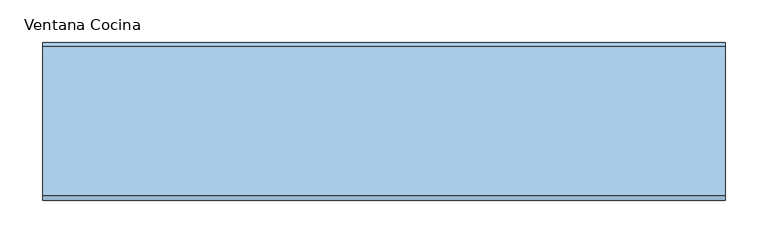
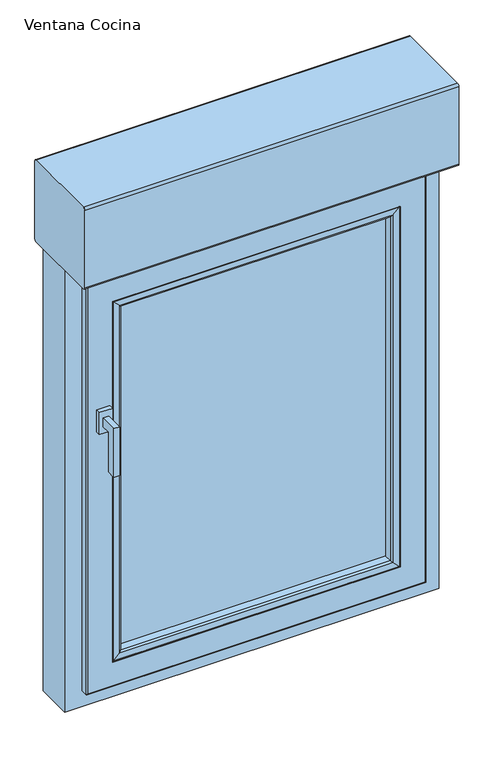
"""IFC4 building model written with IfcOpenShell, lengths in millimetres: window geometry, 2019_ES_Ventana_Replus_re80pvc301_10100_box_1-Hoja_con-Compacto : Ventana Cocina."""

import ifcopenshell
import ifcopenshell.guid

model = None  # the IFC model being written
_history = None  # IfcOwnerHistory: only IFC2X3 demands one
_inside = {}  # id of a spatial element -> (the spatial element, [elements in it])
_under = {}  # id of a project, library or spatial element -> (it, [spatial elements below it])
_declared = {}  # id of a project -> (the project, [libraries it declares])
_typed = {}  # id of a type object -> (the type object, [elements of that type])
_made_of = {}  # id of a material, layer set ... -> (it, [elements and type objects made of it])


def new_model(schema):
    """Start an empty IFC model of exactly this schema.

    Asked for "IFC4X3", IfcOpenShell would pick the latest addendum, in which some entities
    have other attributes; the version numbers below select the first issue.
    IFC2X3 requires an IfcOwnerHistory on every rooted entity: one is made here for all.
    """
    global model, _history
    if schema == "IFC4X3":
        model = ifcopenshell.file(schema_version=(4, 3, 0, 0))
    else:
        model = ifcopenshell.file(schema=schema)
    _inside.clear()
    _under.clear()
    _declared.clear()
    _typed.clear()
    _made_of.clear()
    _history = None
    if model.schema == "IFC2X3":
        org = make("IfcOrganization", Name="unknown")
        user = make(
            "IfcPersonAndOrganization",
            ThePerson=make("IfcPerson", FamilyName="unknown"),
            TheOrganization=org,
        )
        app = make(
            "IfcApplication",
            ApplicationDeveloper=org,
            Version="unknown",
            ApplicationFullName="unknown",
            ApplicationIdentifier="unknown",
        )
        _history = make(
            "IfcOwnerHistory",
            OwningUser=user,
            OwningApplication=app,
            ChangeAction="ADDED",
            CreationDate=0,
        )
    return model


def make(cls, **values):
    """One entity of the class cls with the attributes given. An attribute that is None is left unset."""
    return model.create_entity(
        cls, **{name: value for name, value in values.items() if value is not None}
    )


def rooted(cls, **values):
    """An entity with a GlobalId (a new one), such as an element, a storey or a relation."""
    return make(cls, GlobalId=ifcopenshell.guid.new(), OwnerHistory=_history, **values)


def si_unit(unit_type, name, prefix=None):
    """IfcSIUnit, for example si_unit("LENGTHUNIT", "METRE", prefix="MILLI")."""
    return make("IfcSIUnit", UnitType=unit_type, Prefix=prefix, Name=name)


def assignment(units):
    """IfcUnitAssignment: the units of a project."""
    return None if units is None else make("IfcUnitAssignment", Units=units)


def point(xyz):
    """IfcCartesianPoint."""
    return None if xyz is None else make("IfcCartesianPoint", Coordinates=xyz)


def direction(xyz):
    """IfcDirection."""
    return None if xyz is None else make("IfcDirection", DirectionRatios=xyz)


def frame(location, z_axis=None, x_axis=None):
    """IfcAxis2Placement3D, a coordinate frame: its origin and axes. An axis left out is left unset."""
    return make(
        "IfcAxis2Placement3D",
        Location=point(location),
        Axis=direction(z_axis),
        RefDirection=direction(x_axis),
    )


def frame_2d(location, x_axis=None):
    """IfcAxis2Placement2D, a coordinate frame in the plane: its origin and x axis."""
    return make(
        "IfcAxis2Placement2D", Location=point(location), RefDirection=direction(x_axis)
    )


def origin():
    """The frame at (0, 0, 0) with its axes left unset."""
    return frame((0.0, 0.0, 0.0))


def place(relative_to, where):
    """IfcLocalPlacement: puts the frame where relative to a parent placement (None: the world)."""
    return make(
        "IfcLocalPlacement", PlacementRelTo=relative_to, RelativePlacement=where
    )


def context(
    kind, dimensions, precision=None, world=None, true_north=None, identifier=None
):
    """IfcGeometricRepresentationContext, for example the 3D "Model" context."""
    return make(
        "IfcGeometricRepresentationContext",
        ContextIdentifier=identifier,
        ContextType=kind,
        CoordinateSpaceDimension=dimensions,
        Precision=precision,
        WorldCoordinateSystem=world,
        TrueNorth=true_north,
    )


def project(units=None, contexts=None):
    """IfcProject with its units and contexts."""
    return rooted(
        "IfcProject",
        Name="project",
        RepresentationContexts=contexts,
        UnitsInContext=assignment(units),
    )


def spatial(cls, under=None, at=None, **own):
    """A site, building, storey or space (cls), placed at a placement, below another one or the project."""
    s = rooted(cls, ObjectPlacement=at, **own)
    if under is not None:
        _under.setdefault(under.id(), (under, []))[1].append(s)
    return s


def polyline(points):
    """IfcPolyline through the points."""
    return make("IfcPolyline", Points=[point(p) for p in points])


def circle_curve(where, radius):
    """IfcCircle in the frame where."""
    return make("IfcCircle", Position=where, Radius=radius)


def ellipse_curve(where, semi_axis1, semi_axis2):
    """IfcEllipse in the frame where."""
    return make(
        "IfcEllipse", Position=where, SemiAxis1=semi_axis1, SemiAxis2=semi_axis2
    )


def trimmed(basis, trim1, trim2, sense, master):
    """IfcTrimmedCurve: the piece of a basis curve between two trims."""
    return make(
        "IfcTrimmedCurve",
        BasisCurve=basis,
        Trim1=trim1,
        Trim2=trim2,
        SenseAgreement=sense,
        MasterRepresentation=master,
    )


def segment(curve, same_sense, transition):
    """IfcCompositeCurveSegment."""
    return make(
        "IfcCompositeCurveSegment",
        Transition=transition,
        SameSense=same_sense,
        ParentCurve=curve,
    )


def composite_curve(segments, self_intersect=None):
    """IfcCompositeCurve: segments joined end to end."""
    return make("IfcCompositeCurve", Segments=segments, SelfIntersect=self_intersect)


def outline(outer, holes=None, kind="AREA"):
    """IfcArbitraryClosedProfileDef: a profile drawn as a closed curve; with holes, ...WithVoids."""
    if holes is None:
        return make("IfcArbitraryClosedProfileDef", ProfileType=kind, OuterCurve=outer)
    return make(
        "IfcArbitraryProfileDefWithVoids",
        ProfileType=kind,
        OuterCurve=outer,
        InnerCurves=holes,
    )


def extrude(swept, where, along, depth):
    """IfcExtrudedAreaSolid: the profile swept, set in the frame where, extruded along a direction by depth."""
    return make(
        "IfcExtrudedAreaSolid",
        SweptArea=swept,
        Position=where,
        ExtrudedDirection=direction(along),
        Depth=depth,
    )


def shape(context_of_items, identifier, shape_type, items):
    """IfcShapeRepresentation: the items that make up one representation, for example the "Body"."""
    return make(
        "IfcShapeRepresentation",
        ContextOfItems=context_of_items,
        RepresentationIdentifier=identifier,
        RepresentationType=shape_type,
        Items=items,
    )


def source(mapping_origin, context_of_items, identifier, shape_type, items):
    """IfcRepresentationMap: a shape defined once, which mapped items show again and again."""
    return make(
        "IfcRepresentationMap",
        MappingOrigin=mapping_origin,
        MappedRepresentation=shape(context_of_items, identifier, shape_type, items),
    )


def transform(
    local_origin,
    x_axis=None,
    y_axis=None,
    z_axis=None,
    scale=None,
    scale2=None,
    scale3=None,
    uniform=True,
):
    """IfcCartesianTransformationOperator3D, or its non-uniform kind. x_axis, y_axis, z_axis: its Axis1, 2, 3."""
    if uniform:
        return make(
            "IfcCartesianTransformationOperator3D",
            Axis1=direction(x_axis),
            Axis2=direction(y_axis),
            LocalOrigin=point(local_origin),
            Scale=scale,
            Axis3=direction(z_axis),
        )
    return make(
        "IfcCartesianTransformationOperator3DnonUniform",
        Axis1=direction(x_axis),
        Axis2=direction(y_axis),
        LocalOrigin=point(local_origin),
        Scale=scale,
        Axis3=direction(z_axis),
        Scale2=scale2,
        Scale3=scale3,
    )


def mapped(mapping_source, mapping_target):
    """IfcMappedItem: shows the shape of a source again, moved by a transform."""
    return make(
        "IfcMappedItem", MappingSource=mapping_source, MappingTarget=mapping_target
    )


def made_of(thing, what):
    """Note that an element or type object is made of a material, layer set ...; save() writes the relation."""
    if what is not None:
        _made_of.setdefault(what.id(), (what, []))[1].append(thing)
    return thing


def element(
    cls,
    number,
    at=None,
    inside=None,
    cuts=None,
    type_object=None,
    material=None,
    context=None,
    identifier="Body",
    shape_type=None,
    held_by="IfcProductDefinitionShape",
    body=None,
    shapes=None,
    **own,
):
    """One element of the class cls, such as IfcWall. Its Tag is "e" and its number.

    at: its placement. inside: the storey or other place that contains it. cuts: it is an
    opening in that element (IfcRelVoidsElement). A single representation is given by context,
    identifier, shape_type and body (its items); several are given by shapes. held_by: the class
    of the entity that holds the representations. save() writes the other relations.
    """
    e = rooted(cls, Tag="e%d" % number, ObjectPlacement=at, **own)
    if body is not None:
        shapes = [shape(context, identifier, shape_type, body)]
    if shapes is not None:
        e.Representation = make(held_by, Representations=shapes)
    if inside is not None:
        _inside.setdefault(inside.id(), (inside, []))[1].append(e)
    if cuts is not None:
        rooted(
            "IfcRelVoidsElement", RelatingBuildingElement=cuts, RelatedOpeningElement=e
        )
    if type_object is not None:
        _typed.setdefault(type_object.id(), (type_object, []))[1].append(e)
    return made_of(e, material)


def aggregate(whole, parts):
    """IfcRelAggregates: a whole, such as a stair, and the parts it consists of."""
    return rooted("IfcRelAggregates", RelatingObject=whole, RelatedObjects=parts)


def save(model, path):
    """Write the relations noted so far, then the file.

    IfcRelAggregates (storeys below a building ...), IfcRelContainedInSpatialStructure (elements
    in a storey), IfcRelDefinesByType, IfcRelAssociatesMaterial and IfcRelDeclares: one each for
    every whole, place, type object, material and project.
    """
    for whole, parts in _under.values():
        aggregate(whole, parts)
    for where, things in _inside.values():
        rooted(
            "IfcRelContainedInSpatialStructure",
            RelatedElements=things,
            RelatingStructure=where,
        )
    for kind, things in _typed.values():
        rooted("IfcRelDefinesByType", RelatedObjects=things, RelatingType=kind)
    for what, things in _made_of.values():
        rooted("IfcRelAssociatesMaterial", RelatedObjects=things, RelatingMaterial=what)
    for by, libraries in _declared.values():
        rooted("IfcRelDeclares", RelatingContext=by, RelatedDefinitions=libraries)
    model.write(path)


def plane_surface(at):
    """IfcPlane: the flat surface through the origin of the frame at, square to its z axis."""
    return make("IfcPlane", Position=at)


def cylinder_surface(at, radius):
    """IfcCylindricalSurface: all points at the distance radius from the z axis of the frame at."""
    return make("IfcCylindricalSurface", Position=at, Radius=radius)


def advanced_brep(points, edges, surfaces, faces):
    """IfcAdvancedBrep: a solid bounded by faces that lie on surfaces and meet in shared edges.

    An edge is (start, end): straight between two places in points (the first is 0);
    or (start, end, curve); or (start, end, curve, False) where it runs against its curve.
    A face is (place in surfaces, loops), or (place, loops, False) where it looks against
    its surface's normal. A loop lists edges by number (the first is 1), with a minus sign
    where the edge is run from its end to its start. The first loop is the outer one.
    """
    corners = [point(p) for p in points]
    vertices = [make("IfcVertexPoint", VertexGeometry=c) for c in corners]
    made = []
    for start, end, *more in edges:
        made.append(
            make(
                "IfcEdgeCurve",
                EdgeStart=vertices[start],
                EdgeEnd=vertices[end],
                EdgeGeometry=more[0] if more else make("IfcPolyline", Points=[corners[start], corners[end]]),
                SameSense=more[1] if len(more) > 1 else True,
            )
        )
    hull = []
    for where, loops, *sense in faces:
        bounds = []
        for j, loop in enumerate(loops):
            ring = [make("IfcOrientedEdge", EdgeElement=made[abs(k) - 1], Orientation=k > 0) for k in loop]
            bounds.append(
                make(
                    "IfcFaceOuterBound" if j == 0 else "IfcFaceBound",
                    Bound=make("IfcEdgeLoop", EdgeList=ring),
                    Orientation=True,
                )
            )
        hull.append(make("IfcAdvancedFace", Bounds=bounds, FaceSurface=surfaces[where], SameSense=sense[0] if sense else True))
    return make("IfcAdvancedBrep", Outer=make("IfcClosedShell", CfsFaces=hull))


def ventana_cocina_c5497abf(model_context):
    return source(origin(), model_context, "Body", "SolidModel", [
        extrude(outline(composite_curve([segment(polyline([(55.0, 1810.0), (-120.0, 1810.0)]), True, "CONTINUOUS"), segment(trimmed(circle_curve(frame_2d((-120.0, 1815.0)), 5.0), [point((-120.0, 1810.0))], [point((-125.0, 1815.0))], False, "CARTESIAN"), True, "CONTINUOUS"), segment(polyline([(-125.0, 1815.0), (-125.0, 1990.0)]), True, "CONTINUOUS"), segment(trimmed(circle_curve(frame_2d((-120.0, 1990.0)), 5.0), [point((-125.0, 1990.0))], [point((-120.0, 1995.0))], False, "CARTESIAN"), True, "CONTINUOUS"), segment(polyline([(-120.0, 1995.0), (55.0, 1995.0)]), True, "CONTINUOUS"), segment(trimmed(circle_curve(frame_2d((55.0, 1990.0)), 5.0), [point((55.0, 1995.0))], [point((60.0, 1990.0))], False, "CARTESIAN"), True, "CONTINUOUS"), segment(polyline([(60.0, 1990.0), (60.0, 1815.0)]), True, "CONTINUOUS"), segment(trimmed(circle_curve(frame_2d((55.0, 1815.0)), 5.0), [point((60.0, 1815.0))], [point((55.0, 1810.0))], False, "CARTESIAN"), True, "CONTINUOUS")], self_intersect=False)), frame((-400.0, 0.0, 0.0), z_axis=(1.0, 0.0, 0.0), x_axis=(0.0, 1.0, 0.0)), (0.0, 0.0, 1.0), 800.0),
        extrude(outline(polyline([(-78.4999991, 1470.0), (-78.4999991, 1450.0), (-98.4999991, 1450.0), (-98.4999991, 1360.0), (-118.4999991, 1360.0), (-118.4999991, 1470.0), (-78.4999991, 1470.0)])), frame((-334.1999993, 0.0, 0.0), z_axis=(1.0, 0.0, 0.0), x_axis=(0.0, 1.0, 0.0)), (0.0, 0.0, 1.0), 12.0),
        extrude(outline(polyline([(-313.9687607, -78.4999991), (-342.4312378, -78.4999991), (-342.4312378, -68.4999991), (-313.9687607, -68.4999991), (-313.9687607, -78.4999991)])), frame((0.0, 0.0, 1435.217127), z_axis=(0.0, 0.0, 1.0), x_axis=(1.0, 0.0, 0.0)), (0.0, 0.0, 1.0), 49.565746),
        extrude(outline(polyline([(1707.2, 297.1999993), (1707.2, -297.1999993), (909.8, -297.1999993), (909.8, 297.1999993), (1707.2, 297.1999993)]), holes=[polyline([(917.8, 289.1999993), (917.8, -289.1999993), (1699.2, -289.1999993), (1699.2, 289.1999993), (917.8, 289.1999993)])]), frame((0.0, -26.9999999, 0.0), z_axis=(0.0, 1.0, 0.0), x_axis=(0.0, 0.0, 1.0)), (0.0, 0.0, 1.0), 16.0),
        extrude(outline(polyline([(1707.1868066, 297.1868058), (1707.1868066, -297.1868058), (909.8131934, -297.1868058), (909.8131934, 297.1868058), (1707.1868066, 297.1868058)]), holes=[polyline([(917.8, 289.1999993), (917.8, -289.1999993), (1699.2, -289.1999993), (1699.2, 289.1999993), (917.8, 289.1999993)])]), frame((0.0, -47.0000001, 0.0), z_axis=(0.0, 1.0, 0.0), x_axis=(0.0, 0.0, 1.0)), (0.0, 0.0, 1.0), 16.0),
        extrude(outline(polyline([(297.1999993, -6.9999997), (297.1999993, -10.9999999), (-297.1999993, -10.9999999), (-297.1999993, -6.9999997), (297.1999993, -6.9999997)])), frame((0.0, 0.0, 903.7946451), z_axis=(0.0, 0.0, 1.0), x_axis=(1.0, 0.0, 0.0)), (0.0, 0.0, 1.0), 809.4053549),
        extrude(outline(polyline([(297.1999993, -26.9999999), (297.1999993, -31.0000001), (-297.1999993, -31.0000001), (-297.1999993, -26.9999999), (297.1999993, -26.9999999)])), frame((0.0, 0.0, 903.7946451), z_axis=(0.0, 0.0, 1.0), x_axis=(1.0, 0.0, 0.0)), (0.0, 0.0, 1.0), 809.4053549),
        extrude(outline(polyline([(297.1999993, -47.0000001), (297.1999993, -51.0000003), (-297.1999993, -51.0000003), (-297.1999993, -47.0000001), (297.1999993, -47.0000001)])), frame((0.0, 0.0, 903.7946451), z_axis=(0.0, 0.0, 1.0), x_axis=(1.0, 0.0, 0.0)), (0.0, 0.0, 1.0), 809.4053549),
        advanced_brep(
        [(287.2913171, 9.2764571, 1697.2913178), (290.1890946, 11.5, 1700.1890953), (290.1890946, 11.5, 919.8109047), (287.2913171, 9.2764571, 922.7086822), (330.1999993, 11.5, 879.8), (-330.1999993, 11.5, 879.8), (-330.1999993, 11.5, 1740.2), (330.1999993, 11.5, 1740.2), (-290.1890946, 11.5, 1700.1890953), (-290.1890946, 11.5, 919.8109047), (-287.2913171, 9.2764571, 922.7086822), (284.1757968, -2.3508228, 1694.1757976), (284.1757968, -2.3508228, 925.8242024), (-284.1757968, -2.3508228, 925.8242024), (284.6739305, -3.0000033, 1694.6739313), (284.6739305, -3.0000033, 925.3260687), (-284.6739305, -3.0000033, 925.3260687), (291.1999993, -3.0000033, 1701.2), (-291.1999993, -3.0000033, 1701.2), (-291.1999993, -3.0000033, 918.8), (291.1999993, -3.0000033, 918.8), (-284.6739305, -3.0000033, 1694.6739313), (291.1999993, -6.9999997, 1701.2), (291.1999993, -6.9999997, 918.8), (-291.1999993, -6.9999997, 918.8), (311.8162192, -6.9999997, 1721.8162199), (-311.8162192, -6.9999997, 1721.8162199), (-311.8162192, -6.9999997, 898.1837801), (311.8162192, -6.9999997, 898.1837801), (-291.1999993, -6.9999997, 1701.2), (309.1999993, -25.6153717, 1719.2), (309.1999993, -25.6153717, 900.8), (-309.1999993, -25.6153717, 900.8), (309.1999993, -56.4999995, 1719.2), (309.1999993, -56.4999995, 900.8), (-309.1999993, -56.4999995, 900.8), (-309.1999993, -56.4999995, 1719.2), (297.1999993, -56.4999995, 1707.2), (-297.1999993, -56.4999995, 1707.2), (-297.1999993, -56.4999995, 912.8), (297.1999993, -56.4999995, 912.8), (297.1999993, -51.0000003, 1707.2), (297.1999993, -51.0000003, 912.8), (-297.1999993, -51.0000003, 912.8), (-297.1999993, -51.0000003, 1707.2), (286.007687, -51.0000003, 1696.0076877), (-286.007687, -51.0000003, 1696.0076877), (-286.007687, -51.0000003, 923.9923123), (286.007687, -51.0000003, 923.9923123), (285.4940999, -51.6693201, 1695.4941006), (285.4940999, -51.6693201, 924.5058994), (-285.4940999, -51.6693201, 924.5058994), (288.8993918, -64.3780426, 1698.8993925), (288.8993918, -64.3780426, 921.1006075), (-288.8993918, -64.3780426, 921.1006075), (292.6234971, -67.3403297, 1702.6234978), (292.6234971, -67.3403297, 917.3765022), (-292.6234971, -67.3403297, 917.3765022), (305.6488427, -67.7951848, 1715.6488434), (305.6488427, -67.7951848, 904.3511566), (-305.6488427, -67.7951848, 904.3511566), (306.1999993, -67.2629391, 1716.2), (306.1999993, -67.2629391, 903.8), (-306.1999993, -67.2629391, 903.8), (307.4370593, -68.4999991, 1717.43706), (307.4370593, -68.4999991, 902.56294), (-307.4370593, -68.4999991, 902.56294), (360.1999993, -68.4999991, 1770.2), (-360.1999993, -68.4999991, 1770.2), (-360.1999993, -68.4999991, 849.8), (360.1999993, -68.4999991, 849.8), (-307.4370593, -68.4999991, 1717.43706), (363.1999993, -65.4999991, 1773.2), (363.1999993, -65.4999991, 846.8), (-363.1999993, -65.4999991, 846.8), (363.1999993, -50.0, 1773.2), (363.1999993, -50.0, 846.8), (-363.1999993, -50.0, 846.8), (-363.1999993, -50.0, 1773.2), (343.1999993, -50.0, 1753.2), (-343.1999993, -50.0, 1753.2), (-343.1999993, -50.0, 866.8), (343.1999993, -50.0, 866.8), (343.1999993, -11.9999991, 866.8), (343.1999993, -11.9999991, 1753.2), (-343.1999993, -11.9999991, 866.8), (-343.1999993, -11.9999991, 1753.2), (330.1999993, -11.9999991, 1740.2), (-330.1999993, -11.9999991, 1740.2), (-330.1999993, -11.9999991, 879.8), (330.1999993, -11.9999991, 879.8), (-287.2913171, 9.2764571, 1697.2913178), (-284.1757968, -2.3508228, 1694.1757976), (-309.1999993, -25.6153717, 1719.2), (-285.4940999, -51.6693201, 1695.4941006), (-288.8993918, -64.3780426, 1698.8993925), (-292.6234971, -67.3403297, 1702.6234978), (-305.6488427, -67.7951848, 1715.6488434), (-306.1999993, -67.2629391, 1716.2), (-363.1999993, -65.4999991, 1773.2)],
        [
            (0, 1, ellipse_curve(frame((290.1890946, 8.5, 1700.1890953), z_axis=(0.7071067811865475, 0.0, -0.7071067811865475), x_axis=(0.7071067811865474, 0.0, 0.7071067811865476)), 4.2426407, 3.0)),
            (1, 2),
            (2, 3, ellipse_curve(frame((290.1890946, 8.5, 919.8109047), z_axis=(0.7071067811865475, 0.0, 0.7071067811865475), x_axis=(-0.7071067811865474, 0.0, 0.7071067811865476)), 4.2426407, 3.0)),
            (3, 0),
            (4, 5),
            (5, 6),
            (6, 7),
            (7, 4),
            (1, 8),
            (8, 9),
            (9, 2),
            (9, 10, ellipse_curve(frame((-290.1890946, 8.5, 919.8109047), z_axis=(0.7071067811865475, 0.0, -0.7071067811865475), x_axis=(0.7071067811865476, 0.0, 0.7071067811865474)), 4.2426407, 3.0)),
            (10, 3),
            (11, 0),
            (3, 12),
            (12, 11),
            (10, 13),
            (13, 12),
            (14, 11, ellipse_curve(frame((284.6739305, -2.4842973, 1694.6739313), z_axis=(0.7071067811865475, 0.0, -0.7071067811865475), x_axis=(0.7071067811865474, 0.0, 0.7071067811865476)), 0.7293184, 0.515706)),
            (12, 15, ellipse_curve(frame((284.6739305, -2.4842973, 925.3260687), z_axis=(0.7071067811865475, 0.0, 0.7071067811865475), x_axis=(-0.7071067811865474, 0.0, 0.7071067811865476)), 0.7293184, 0.515706)),
            (15, 14),
            (13, 16, ellipse_curve(frame((-284.6739305, -2.4842973, 925.3260687), z_axis=(0.7071067811865475, 0.0, -0.7071067811865475), x_axis=(0.7071067811865476, 0.0, 0.7071067811865474)), 0.7293184, 0.515706)),
            (16, 15),
            (17, 18),
            (18, 19),
            (19, 20),
            (20, 17),
            (16, 21),
            (21, 14),
            (22, 17),
            (20, 23),
            (23, 22),
            (19, 24),
            (24, 23),
            (25, 26),
            (26, 27),
            (27, 28),
            (28, 25),
            (24, 29),
            (29, 22),
            (30, 25),
            (28, 31),
            (31, 30),
            (27, 32),
            (32, 31),
            (33, 30),
            (31, 34),
            (34, 33),
            (32, 35),
            (35, 34),
            (35, 36),
            (36, 33),
            (37, 38),
            (38, 39),
            (39, 40),
            (40, 37),
            (41, 37),
            (40, 42),
            (42, 41),
            (39, 43),
            (43, 42),
            (43, 44),
            (44, 41),
            (45, 46),
            (46, 47),
            (47, 48),
            (48, 45),
            (49, 45, ellipse_curve(frame((286.007687, -51.5317048, 1696.0076877), z_axis=(0.7071067811865475, 0.0, -0.7071067811865475), x_axis=(0.7071067811865474, 0.0, 0.7071067811865476)), 0.7519437, 0.5317045)),
            (48, 50, ellipse_curve(frame((286.007687, -51.5317048, 923.9923123), z_axis=(0.7071067811865475, 0.0, 0.7071067811865475), x_axis=(-0.7071067811865474, 0.0, 0.7071067811865476)), 0.7519437, 0.5317045)),
            (50, 49),
            (47, 51, ellipse_curve(frame((-286.007687, -51.5317048, 923.9923123), z_axis=(0.7071067811865475, 0.0, -0.7071067811865475), x_axis=(0.7071067811865476, 0.0, 0.7071067811865474)), 0.7519437, 0.5317045)),
            (51, 50),
            (52, 49),
            (50, 53),
            (53, 52),
            (51, 54),
            (54, 53),
            (55, 52, ellipse_curve(frame((292.7630951, -63.3427664, 1702.7630958), z_axis=(0.7071067811865475, 0.0, -0.7071067811865475), x_axis=(0.7071067811865474, 0.0, 0.7071067811865476)), 5.6568542, 4.0)),
            (53, 56, ellipse_curve(frame((292.7630951, -63.3427664, 917.2369042), z_axis=(0.7071067811865475, 0.0, 0.7071067811865475), x_axis=(-0.7071067811865474, 0.0, 0.7071067811865476)), 5.6568542, 4.0)),
            (56, 55),
            (54, 57, ellipse_curve(frame((-292.7630951, -63.3427664, 917.2369042), z_axis=(0.7071067811865475, 0.0, -0.7071067811865475), x_axis=(0.7071067811865476, 0.0, 0.7071067811865474)), 5.6568542, 4.0)),
            (57, 56),
            (58, 55),
            (56, 59),
            (59, 58),
            (57, 60),
            (60, 59),
            (61, 58, ellipse_curve(frame((305.6674291, -67.2629391, 1715.6674299), z_axis=(0.7071067811865475, 0.0, -0.7071067811865475), x_axis=(0.7071067811865474, 0.0, 0.7071067811865476)), 0.7531679, 0.5325701)),
            (59, 62, ellipse_curve(frame((305.6674291, -67.2629391, 904.3325701), z_axis=(0.7071067811865475, 0.0, 0.7071067811865475), x_axis=(-0.7071067811865474, 0.0, 0.7071067811865476)), 0.7531679, 0.5325701)),
            (62, 61),
            (60, 63, ellipse_curve(frame((-305.6674291, -67.2629391, 904.3325701), z_axis=(0.7071067811865475, 0.0, -0.7071067811865475), x_axis=(0.7071067811865476, 0.0, 0.7071067811865474)), 0.7531679, 0.5325701)),
            (63, 62),
            (64, 61, ellipse_curve(frame((307.4370593, -67.2629391, 1717.43706), z_axis=(0.7071067811865475, 0.0, -0.7071067811865475), x_axis=(0.7071067811865474, 0.0, 0.7071067811865476)), 1.7494671, 1.23706)),
            (62, 65, ellipse_curve(frame((307.4370593, -67.2629391, 902.56294), z_axis=(0.7071067811865475, 0.0, 0.7071067811865475), x_axis=(-0.7071067811865474, 0.0, 0.7071067811865476)), 1.7494671, 1.23706)),
            (65, 64),
            (63, 66, ellipse_curve(frame((-307.4370593, -67.2629391, 902.56294), z_axis=(0.7071067811865475, 0.0, -0.7071067811865475), x_axis=(0.7071067811865476, 0.0, 0.7071067811865474)), 1.7494671, 1.23706)),
            (66, 65),
            (67, 68),
            (68, 69),
            (69, 70),
            (70, 67),
            (66, 71),
            (71, 64),
            (72, 67, ellipse_curve(frame((360.1999993, -65.4999991, 1770.2), z_axis=(0.7071067811865475, 0.0, -0.7071067811865475), x_axis=(0.7071067811865474, 0.0, 0.7071067811865476)), 4.2426407, 3.0)),
            (70, 73, ellipse_curve(frame((360.1999993, -65.4999991, 849.8), z_axis=(0.7071067811865475, 0.0, 0.7071067811865475), x_axis=(-0.7071067811865474, 0.0, 0.7071067811865476)), 4.2426407, 3.0)),
            (73, 72),
            (69, 74, ellipse_curve(frame((-360.1999993, -65.4999991, 849.8), z_axis=(0.7071067811865475, 0.0, -0.7071067811865475), x_axis=(0.7071067811865476, 0.0, 0.7071067811865474)), 4.2426407, 3.0)),
            (74, 73),
            (75, 72),
            (73, 76),
            (76, 75),
            (74, 77),
            (77, 76),
            (77, 78),
            (78, 75),
            (79, 80),
            (80, 81),
            (81, 82),
            (82, 79),
            (82, 83),
            (83, 84),
            (84, 79),
            (81, 85),
            (85, 83),
            (85, 86),
            (86, 84),
            (87, 88),
            (88, 89),
            (89, 90),
            (90, 87),
            (90, 4),
            (7, 87),
            (89, 5),
            (8, 91, ellipse_curve(frame((-290.1890946, 8.5, 1700.1890953), z_axis=(-0.7071067811865475, 0.0, -0.7071067811865475), x_axis=(0.7071067811865474, 0.0, -0.7071067811865476)), 4.2426407, 3.0)),
            (91, 10),
            (91, 92),
            (92, 13),
            (92, 21, ellipse_curve(frame((-284.6739305, -2.4842973, 1694.6739313), z_axis=(-0.7071067811865475, 0.0, -0.7071067811865475), x_axis=(0.7071067811865474, 0.0, -0.7071067811865476)), 0.7293184, 0.515706)),
            (18, 29),
            (26, 93),
            (93, 32),
            (93, 36),
            (38, 44),
            (46, 94, ellipse_curve(frame((-286.007687, -51.5317048, 1696.0076877), z_axis=(-0.7071067811865475, 0.0, -0.7071067811865475), x_axis=(0.7071067811865474, 0.0, -0.7071067811865476)), 0.7519437, 0.5317045)),
            (94, 51),
            (94, 95),
            (95, 54),
            (95, 96, ellipse_curve(frame((-292.7630951, -63.3427664, 1702.7630958), z_axis=(-0.7071067811865475, 0.0, -0.7071067811865475), x_axis=(0.7071067811865474, 0.0, -0.7071067811865476)), 5.6568542, 4.0)),
            (96, 57),
            (96, 97),
            (97, 60),
            (97, 98, ellipse_curve(frame((-305.6674291, -67.2629391, 1715.6674299), z_axis=(-0.7071067811865475, 0.0, -0.7071067811865475), x_axis=(0.7071067811865474, 0.0, -0.7071067811865476)), 0.7531679, 0.5325701)),
            (98, 63),
            (98, 71, ellipse_curve(frame((-307.4370593, -67.2629391, 1717.43706), z_axis=(-0.7071067811865475, 0.0, -0.7071067811865475), x_axis=(0.7071067811865474, 0.0, -0.7071067811865476)), 1.7494671, 1.23706)),
            (68, 99, ellipse_curve(frame((-360.1999993, -65.4999991, 1770.2), z_axis=(-0.7071067811865475, 0.0, -0.7071067811865475), x_axis=(0.7071067811865474, 0.0, -0.7071067811865476)), 4.2426407, 3.0)),
            (99, 74),
            (99, 78),
            (80, 86),
            (88, 6),
            (0, 91),
            (11, 92),
            (30, 93),
            (49, 94),
            (52, 95),
            (55, 96),
            (58, 97),
            (61, 98),
            (72, 99),
        ],
        [
            cylinder_surface(frame((290.1890946, 8.5, 1773.2), z_axis=(0.0, 0.0, 1.0), x_axis=(-1.0, 0.0, 0.0)), 3.0),
            plane_surface(frame((-330.1999993, 11.5, 1740.2), z_axis=(0.0, 1.0, 0.0), x_axis=(1.0, 0.0, 0.0))),
            cylinder_surface(frame((363.1999993, 8.5, 919.8109047), z_axis=(1.0, 0.0, 0.0), x_axis=(0.0, 0.0, 1.0)), 3.0),
            plane_surface(frame((287.2913171, 9.2764571, 1697.2913178), z_axis=(-0.9659258263570556, 0.258819044848789, 0.0), x_axis=(0.0, 0.0, -1.0))),
            plane_surface(frame((287.2913171, 9.2764571, 922.7086822), z_axis=(0.0, 0.2588190448487859, 0.9659258263570565), x_axis=(-1.0, 0.0, 0.0))),
            cylinder_surface(frame((284.6739305, -2.4842973, 1773.2), z_axis=(0.0, 0.0, 1.0), x_axis=(-1.0, 0.0, 0.0)), 0.515706),
            cylinder_surface(frame((363.1999993, -2.4842973, 925.3260687), z_axis=(1.0, 0.0, 0.0), x_axis=(0.0, 0.0, 1.0)), 0.515706),
            plane_surface(frame((-284.6739305, -3.0000033, 1694.6739313), z_axis=(0.0, -1.0, 0.0), x_axis=(1.0, 0.0, 0.0))),
            plane_surface(frame((291.1999993, -3.0000033, 1701.2), z_axis=(-1.0, 0.0, 0.0), x_axis=(0.0, 0.0, -1.0))),
            plane_surface(frame((291.1999993, -3.0000033, 918.8), z_axis=(0.0, 0.0, 1.0), x_axis=(-1.0, 0.0, 0.0))),
            plane_surface(frame((-291.1999993, -6.9999997, 1701.2), z_axis=(0.0, -1.0, 0.0), x_axis=(1.0, 0.0, 0.0))),
            plane_surface(frame((311.8162192, -6.9999997, 1721.8162199), z_axis=(-0.9902680687415736, 0.13917310096004265, 0.0), x_axis=(0.0, 0.0, -1.0))),
            plane_surface(frame((311.8162192, -6.9999997, 898.1837801), z_axis=(0.0, 0.13917310096003943, 0.990268068741574), x_axis=(-1.0, 0.0, 0.0))),
            plane_surface(frame((309.1999993, -25.6153717, 1719.2), z_axis=(-1.0, 0.0, 0.0), x_axis=(0.0, 0.0, -1.0))),
            plane_surface(frame((309.1999993, -25.6153717, 900.8), z_axis=(0.0, 0.0, 1.0), x_axis=(-1.0, 0.0, 0.0))),
            plane_surface(frame((-309.1999993, -56.4999995, 1719.2), z_axis=(0.0, 1.0, 0.0), x_axis=(1.0, 0.0, 0.0))),
            plane_surface(frame((297.1999993, -56.4999995, 1707.2), z_axis=(1.0, 0.0, 0.0), x_axis=(0.0, 0.0, -1.0))),
            plane_surface(frame((297.1999993, -56.4999995, 912.8), z_axis=(0.0, 0.0, -1.0), x_axis=(-1.0, 0.0, 0.0))),
            plane_surface(frame((-297.1999993, -51.0000003, 1707.2), z_axis=(0.0, 1.0, 0.0), x_axis=(1.0, 0.0, 0.0))),
            cylinder_surface(frame((286.007687, -51.5317048, 1773.2), z_axis=(0.0, 0.0, 1.0), x_axis=(-1.0, 0.0, 0.0)), 0.5317045),
            cylinder_surface(frame((363.1999993, -51.5317048, 923.9923123), z_axis=(1.0, 0.0, 0.0), x_axis=(0.0, 0.0, 1.0)), 0.5317045),
            plane_surface(frame((285.4940999, -51.6693201, 1695.4941006), z_axis=(-0.9659258262890666, -0.2588190451025272, 0.0), x_axis=(0.0, 0.0, -1.0))),
            plane_surface(frame((285.4940999, -51.6693201, 924.5058994), z_axis=(0.0, -0.2588190451025303, 0.9659258262890658), x_axis=(-1.0, 0.0, 0.0))),
            cylinder_surface(frame((292.7630951, -63.3427664, 1773.2), z_axis=(0.0, 0.0, 1.0), x_axis=(-1.0, 0.0, 0.0)), 4.0),
            cylinder_surface(frame((363.1999993, -63.3427664, 917.2369042), z_axis=(1.0, 0.0, 0.0), x_axis=(0.0, 0.0, 1.0)), 4.0),
            plane_surface(frame((292.6234971, -67.3403297, 1702.6234978), z_axis=(-0.03489949670250791, -0.9993908270190955, 0.0), x_axis=(0.0, 0.0, -1.0))),
            plane_surface(frame((292.6234971, -67.3403297, 917.3765022), z_axis=(0.0, -0.9993908270190957, 0.034899496702504675), x_axis=(-1.0, 0.0, 0.0))),
            cylinder_surface(frame((305.6674291, -67.2629391, 1773.2), z_axis=(0.0, 0.0, 1.0), x_axis=(-1.0, 0.0, 0.0)), 0.5325701),
            cylinder_surface(frame((363.1999993, -67.2629391, 904.3325701), z_axis=(1.0, 0.0, 0.0), x_axis=(0.0, 0.0, 1.0)), 0.5325701),
            cylinder_surface(frame((307.4370593, -67.2629391, 1773.2), z_axis=(0.0, 0.0, 1.0), x_axis=(-1.0, 0.0, 0.0)), 1.23706),
            cylinder_surface(frame((363.1999993, -67.2629391, 902.56294), z_axis=(1.0, 0.0, 0.0), x_axis=(0.0, 0.0, 1.0)), 1.23706),
            plane_surface(frame((-307.4370593, -68.4999991, 1717.43706), z_axis=(0.0, -1.0, 0.0), x_axis=(1.0, 0.0, 0.0))),
            cylinder_surface(frame((360.1999993, -65.4999991, 1773.2), z_axis=(0.0, 0.0, 1.0), x_axis=(-1.0, 0.0, 0.0)), 3.0),
            cylinder_surface(frame((363.1999993, -65.4999991, 849.8), z_axis=(1.0, 0.0, 0.0), x_axis=(0.0, 0.0, 1.0)), 3.0),
            plane_surface(frame((363.1999993, -65.4999991, 1773.2), z_axis=(1.0, 0.0, 0.0), x_axis=(0.0, 0.0, -1.0))),
            plane_surface(frame((363.1999993, -65.4999991, 846.8), z_axis=(0.0, 0.0, -1.0), x_axis=(-1.0, 0.0, 0.0))),
            plane_surface(frame((-359.2000019, -50.0, 1769.2000027), z_axis=(0.0, 1.0, 0.0), x_axis=(1.0, 0.0, 0.0))),
            plane_surface(frame((343.1999993, -45.0999991, 1753.2), z_axis=(1.0, 0.0, 0.0), x_axis=(0.0, 0.0, -1.0))),
            plane_surface(frame((343.1999993, -45.0999991, 866.8), z_axis=(0.0, 0.0, -1.0), x_axis=(-1.0, 0.0, 0.0))),
            plane_surface(frame((-335.7000002, -11.9999991, 1745.7000009), z_axis=(0.0, 1.0, 0.0), x_axis=(1.0, 0.0, 0.0))),
            plane_surface(frame((330.1999993, -1.4999991, 1740.2), z_axis=(1.0, 0.0, 0.0), x_axis=(0.0, 0.0, -1.0))),
            plane_surface(frame((330.1999993, -1.4999991, 879.8), z_axis=(0.0, 0.0, -1.0), x_axis=(-1.0, 0.0, 0.0))),
            cylinder_surface(frame((-290.1890946, 8.5, 846.8), z_axis=(0.0, 0.0, -1.0), x_axis=(1.0, 0.0, 0.0)), 3.0),
            plane_surface(frame((-287.2913171, 9.2764571, 922.7086822), z_axis=(0.9659258263570573, 0.25881904484878276, 0.0), x_axis=(0.0, 0.0, 1.0))),
            cylinder_surface(frame((-284.6739305, -2.4842973, 846.8), z_axis=(0.0, 0.0, -1.0), x_axis=(1.0, 0.0, 0.0)), 0.515706),
            plane_surface(frame((-291.1999993, -3.0000033, 918.8), z_axis=(1.0, 0.0, 0.0), x_axis=(0.0, 0.0, 1.0))),
            plane_surface(frame((-311.8162192, -6.9999997, 898.1837801), z_axis=(0.9902680687415745, 0.1391731009600362, 0.0), x_axis=(0.0, 0.0, 1.0))),
            plane_surface(frame((-309.1999993, -25.6153717, 900.8), z_axis=(1.0, 0.0, 0.0), x_axis=(0.0, 0.0, 1.0))),
            plane_surface(frame((-297.1999993, -56.4999995, 912.8), z_axis=(-1.0, 0.0, 0.0), x_axis=(0.0, 0.0, 1.0))),
            cylinder_surface(frame((-286.007687, -51.5317048, 846.8), z_axis=(0.0, 0.0, -1.0), x_axis=(1.0, 0.0, 0.0)), 0.5317045),
            plane_surface(frame((-285.4940999, -51.6693201, 924.5058994), z_axis=(0.9659258262890649, -0.2588190451025334, 0.0), x_axis=(0.0, 0.0, 1.0))),
            cylinder_surface(frame((-292.7630951, -63.3427664, 846.8), z_axis=(0.0, 0.0, -1.0), x_axis=(1.0, 0.0, 0.0)), 4.0),
            plane_surface(frame((-292.6234971, -67.3403297, 917.3765022), z_axis=(0.03489949670250144, -0.9993908270190958, 0.0), x_axis=(0.0, 0.0, 1.0))),
            cylinder_surface(frame((-305.6674291, -67.2629391, 846.8), z_axis=(0.0, 0.0, -1.0), x_axis=(1.0, 0.0, 0.0)), 0.5325701),
            cylinder_surface(frame((-307.4370593, -67.2629391, 846.8), z_axis=(0.0, 0.0, -1.0), x_axis=(1.0, 0.0, 0.0)), 1.23706),
            cylinder_surface(frame((-360.1999993, -65.4999991, 846.8), z_axis=(0.0, 0.0, -1.0), x_axis=(1.0, 0.0, 0.0)), 3.0),
            plane_surface(frame((-363.1999993, -65.4999991, 846.8), z_axis=(-1.0, 0.0, 0.0), x_axis=(0.0, 0.0, 1.0))),
            plane_surface(frame((-343.1999993, -45.0999991, 866.8), z_axis=(-1.0, 0.0, 0.0), x_axis=(0.0, 0.0, 1.0))),
            plane_surface(frame((-330.1999993, -1.4999991, 879.8), z_axis=(-1.0, 0.0, 0.0), x_axis=(0.0, 0.0, 1.0))),
            cylinder_surface(frame((-363.1999993, 8.5, 1700.1890953), z_axis=(-1.0, 0.0, 0.0), x_axis=(0.0, 0.0, -1.0)), 3.0),
            plane_surface(frame((-287.2913171, 9.2764571, 1697.2913178), z_axis=(0.0, 0.2588190448487859, -0.9659258263570564), x_axis=(1.0, 0.0, 0.0))),
            cylinder_surface(frame((-363.1999993, -2.4842973, 1694.6739313), z_axis=(-1.0, 0.0, 0.0), x_axis=(0.0, 0.0, -1.0)), 0.515706),
            plane_surface(frame((-291.1999993, -3.0000033, 1701.2), z_axis=(0.0, 0.0, -1.0), x_axis=(1.0, 0.0, 0.0))),
            plane_surface(frame((-311.8162192, -6.9999997, 1721.8162199), z_axis=(0.0, 0.13917310096003943, -0.990268068741574), x_axis=(1.0, 0.0, 0.0))),
            plane_surface(frame((-309.1999993, -25.6153717, 1719.2), z_axis=(0.0, 0.0, -1.0), x_axis=(1.0, 0.0, 0.0))),
            plane_surface(frame((-297.1999993, -56.4999995, 1707.2), z_axis=(0.0, 0.0, 1.0), x_axis=(1.0, 0.0, 0.0))),
            cylinder_surface(frame((-363.1999993, -51.5317048, 1696.0076877), z_axis=(-1.0, 0.0, 0.0), x_axis=(0.0, 0.0, -1.0)), 0.5317045),
            plane_surface(frame((-285.4940999, -51.6693201, 1695.4941006), z_axis=(0.0, -0.2588190451025303, -0.9659258262890658), x_axis=(1.0, 0.0, 0.0))),
            cylinder_surface(frame((-363.1999993, -63.3427664, 1702.7630958), z_axis=(-1.0, 0.0, 0.0), x_axis=(0.0, 0.0, -1.0)), 4.0),
            plane_surface(frame((-292.6234971, -67.3403297, 1702.6234978), z_axis=(0.0, -0.9993908270190957, -0.034899496702504675), x_axis=(1.0, 0.0, 0.0))),
            cylinder_surface(frame((-363.1999993, -67.2629391, 1715.6674299), z_axis=(-1.0, 0.0, 0.0), x_axis=(0.0, 0.0, -1.0)), 0.5325701),
            cylinder_surface(frame((-363.1999993, -67.2629391, 1717.43706), z_axis=(-1.0, 0.0, 0.0), x_axis=(0.0, 0.0, -1.0)), 1.23706),
            cylinder_surface(frame((-363.1999993, -65.4999991, 1770.2), z_axis=(-1.0, 0.0, 0.0), x_axis=(0.0, 0.0, -1.0)), 3.0),
            plane_surface(frame((-363.1999993, -65.4999991, 1773.2), z_axis=(0.0, 0.0, 1.0), x_axis=(1.0, 0.0, 0.0))),
            plane_surface(frame((-343.1999993, -45.0999991, 1753.2), z_axis=(0.0, 0.0, 1.0), x_axis=(1.0, 0.0, 0.0))),
            plane_surface(frame((-330.1999993, -1.4999991, 1740.2), z_axis=(0.0, 0.0, 1.0), x_axis=(1.0, 0.0, 0.0))),
        ],
        [
            (0, [[1, 2, 3, 4]]),
            (1, [[5, 6, 7, 8], [9, 10, 11, -2]]),
            (2, [[-3, -11, 12, 13]]),
            (3, [[14, -4, 15, 16]]),
            (4, [[-15, -13, 17, 18]]),
            (5, [[19, -16, 20, 21]]),
            (6, [[-20, -18, 22, 23]]),
            (7, [[24, 25, 26, 27], [-23, 28, 29, -21]]),
            (8, [[30, -27, 31, 32]]),
            (9, [[-31, -26, 33, 34]]),
            (10, [[35, 36, 37, 38], [-34, 39, 40, -32]]),
            (11, [[41, -38, 42, 43]]),
            (12, [[-42, -37, 44, 45]]),
            (13, [[46, -43, 47, 48]]),
            (14, [[-47, -45, 49, 50]]),
            (15, [[-50, 51, 52, -48], [53, 54, 55, 56]]),
            (16, [[57, -56, 58, 59]]),
            (17, [[-58, -55, 60, 61]]),
            (18, [[-61, 62, 63, -59], [64, 65, 66, 67]]),
            (19, [[68, -67, 69, 70]]),
            (20, [[-69, -66, 71, 72]]),
            (21, [[73, -70, 74, 75]]),
            (22, [[-74, -72, 76, 77]]),
            (23, [[78, -75, 79, 80]]),
            (24, [[-79, -77, 81, 82]]),
            (25, [[83, -80, 84, 85]]),
            (26, [[-84, -82, 86, 87]]),
            (27, [[88, -85, 89, 90]]),
            (28, [[-89, -87, 91, 92]]),
            (29, [[93, -90, 94, 95]]),
            (30, [[-94, -92, 96, 97]]),
            (31, [[98, 99, 100, 101], [-97, 102, 103, -95]]),
            (32, [[104, -101, 105, 106]]),
            (33, [[-105, -100, 107, 108]]),
            (34, [[109, -106, 110, 111]]),
            (35, [[-110, -108, 112, 113]]),
            (36, [[-113, 114, 115, -111], [116, 117, 118, 119]]),
            (37, [[-119, 120, 121, 122]]),
            (38, [[-120, -118, 123, 124]]),
            (39, [[-124, 125, 126, -121], [127, 128, 129, 130]]),
            (40, [[-130, 131, -8, 132]]),
            (41, [[-131, -129, 133, -5]]),
            (42, [[-12, -10, 134, 135]]),
            (43, [[-17, -135, 136, 137]]),
            (44, [[-22, -137, 138, -28]]),
            (45, [[-33, -25, 139, -39]]),
            (46, [[-44, -36, 140, 141]]),
            (47, [[-49, -141, 142, -51]]),
            (48, [[-60, -54, 143, -62]]),
            (49, [[-71, -65, 144, 145]]),
            (50, [[-76, -145, 146, 147]]),
            (51, [[-81, -147, 148, 149]]),
            (52, [[-86, -149, 150, 151]]),
            (53, [[-91, -151, 152, 153]]),
            (54, [[-96, -153, 154, -102]]),
            (55, [[-107, -99, 155, 156]]),
            (56, [[-112, -156, 157, -114]]),
            (57, [[-123, -117, 158, -125]]),
            (58, [[-133, -128, 159, -6]]),
            (59, [[-134, -9, -1, 160]]),
            (60, [[-136, -160, -14, 161]]),
            (61, [[-138, -161, -19, -29]]),
            (62, [[-139, -24, -30, -40]]),
            (63, [[-140, -35, -41, 162]]),
            (64, [[-142, -162, -46, -52]]),
            (65, [[-143, -53, -57, -63]]),
            (66, [[-144, -64, -68, 163]]),
            (67, [[-146, -163, -73, 164]]),
            (68, [[-148, -164, -78, 165]]),
            (69, [[-150, -165, -83, 166]]),
            (70, [[-152, -166, -88, 167]]),
            (71, [[-154, -167, -93, -103]]),
            (72, [[-155, -98, -104, 168]]),
            (73, [[-157, -168, -109, -115]]),
            (74, [[-158, -116, -122, -126]]),
            (75, [[-159, -127, -132, -7]]),
        ],
    ),
        advanced_brep(
        [(323.2673545, 12.758819, 1733.2673545), (327.2913185, 27.7764571, 1737.2913185), (327.2913185, 27.7764571, 882.7086815), (323.2673545, 12.758819, 886.7326455), (330.189096, 30.0, 1740.189096), (330.189096, 30.0, 879.810904), (-327.2913185, 27.7764571, 882.7086815), (-323.2673545, 12.758819, 886.7326455), (324.2332803, 11.5, 1734.2332803), (324.2332803, 11.5, 885.7667197), (400.0, 30.0, 1810.0), (400.0, -50.0, 1810.0), (400.0, -50.0, 810.0), (400.0, 30.0, 810.0), (-400.0, -50.0, 1810.0), (-400.0, -50.0, 810.0), (356.1999993, -50.0, 853.8000007), (-356.1999993, -50.0, 853.8000007), (-356.1999993, -50.0, 1766.1999993), (356.1999993, -50.0, 1766.1999993), (-400.0, 30.0, 810.0), (-400.0, 30.0, 1810.0), (-330.189096, 30.0, 1740.189096), (-330.189096, 30.0, 879.810904), (336.1891471, -8.0, 1746.1891471), (336.1891471, 11.5, 1746.1891471), (336.1891471, 11.5, 873.8108529), (336.1891471, -8.0, 873.8108529), (-336.1891471, 11.5, 1746.1891471), (-336.1891471, 11.5, 873.8108529), (-324.2332803, 11.5, 885.7667197), (-324.2332803, 11.5, 1734.2332803), (-336.1891471, -8.0, 873.8108529), (355.1999993, -8.0, 1765.1999993), (-355.1999993, -8.0, 1765.1999993), (-355.1999993, -8.0, 854.8000007), (355.1999993, -8.0, 854.8000007), (-336.1891471, -8.0, 1746.1891471), (355.1999993, -49.0, 1765.1999993), (355.1999993, -49.0, 854.8000007), (-355.1999993, -49.0, 854.8000007), (-327.2913185, 27.7764571, 1737.2913185), (-323.2673545, 12.758819, 1733.2673545), (-355.1999993, -49.0, 1765.1999993)],
        [
            (0, 1),
            (1, 2),
            (2, 3),
            (3, 0),
            (1, 4, ellipse_curve(frame((330.189096, 27.0, 1740.189096), z_axis=(0.7071067811865475, 0.0, -0.7071067811865475), x_axis=(0.7071067811865474, 0.0, 0.7071067811865476)), 4.2426407, 3.0)),
            (4, 5),
            (5, 2, ellipse_curve(frame((330.189096, 27.0, 879.810904), z_axis=(0.7071067811865475, 0.0, 0.7071067811865475), x_axis=(-0.7071067811865474, 0.0, 0.7071067811865476)), 4.2426407, 3.0)),
            (2, 6),
            (6, 7),
            (7, 3),
            (8, 0, ellipse_curve(frame((324.2332803, 12.5, 1734.2332803), z_axis=(0.7071067811865475, 0.0, -0.7071067811865475), x_axis=(0.7071067811865474, 0.0, 0.7071067811865476)), 1.4142136, 1.0)),
            (3, 9, ellipse_curve(frame((324.2332803, 12.5, 885.7667197), z_axis=(0.7071067811865475, 0.0, 0.7071067811865475), x_axis=(-0.7071067811865474, 0.0, 0.7071067811865476)), 1.4142136, 1.0)),
            (9, 8),
            (10, 11),
            (11, 12),
            (12, 13),
            (13, 10),
            (11, 14),
            (14, 15),
            (15, 12),
            (16, 17),
            (17, 18),
            (18, 19),
            (19, 16),
            (15, 20),
            (20, 13),
            (20, 21),
            (21, 10),
            (4, 22),
            (22, 23),
            (23, 5),
            (24, 25),
            (25, 26),
            (26, 27),
            (27, 24),
            (25, 28),
            (28, 29),
            (29, 26),
            (9, 30),
            (30, 31),
            (31, 8),
            (29, 32),
            (32, 27),
            (33, 34),
            (34, 35),
            (35, 36),
            (36, 33),
            (32, 37),
            (37, 24),
            (19, 38, ellipse_curve(frame((356.1999993, -49.0, 1766.1999993), z_axis=(0.7071067811865475, 0.0, -0.7071067811865475), x_axis=(0.7071067811865474, 0.0, 0.7071067811865476)), 1.4142136, 1.0)),
            (38, 39),
            (39, 16, ellipse_curve(frame((356.1999993, -49.0, 853.8000007), z_axis=(0.7071067811865475, 0.0, 0.7071067811865475), x_axis=(-0.7071067811865474, 0.0, 0.7071067811865476)), 1.4142136, 1.0)),
            (38, 33),
            (36, 39),
            (39, 40),
            (40, 17, ellipse_curve(frame((-356.1999993, -49.0, 853.8000007), z_axis=(0.7071067811865475, 0.0, -0.7071067811865475), x_axis=(0.7071067811865476, 0.0, 0.7071067811865474)), 1.4142136, 1.0)),
            (7, 30, ellipse_curve(frame((-324.2332803, 12.5, 885.7667197), z_axis=(0.7071067811865475, 0.0, -0.7071067811865475), x_axis=(0.7071067811865476, 0.0, 0.7071067811865474)), 1.4142136, 1.0)),
            (23, 6, ellipse_curve(frame((-330.189096, 27.0, 879.810904), z_axis=(0.7071067811865475, 0.0, -0.7071067811865475), x_axis=(0.7071067811865476, 0.0, 0.7071067811865474)), 4.2426407, 3.0)),
            (6, 41),
            (41, 42),
            (42, 7),
            (14, 21),
            (28, 37),
            (35, 40),
            (40, 43),
            (43, 18, ellipse_curve(frame((-356.1999993, -49.0, 1766.1999993), z_axis=(-0.7071067811865475, 0.0, -0.7071067811865475), x_axis=(0.7071067811865474, 0.0, -0.7071067811865476)), 1.4142136, 1.0)),
            (42, 31, ellipse_curve(frame((-324.2332803, 12.5, 1734.2332803), z_axis=(-0.7071067811865475, 0.0, -0.7071067811865475), x_axis=(0.7071067811865474, 0.0, -0.7071067811865476)), 1.4142136, 1.0)),
            (22, 41, ellipse_curve(frame((-330.189096, 27.0, 1740.189096), z_axis=(-0.7071067811865475, 0.0, -0.7071067811865475), x_axis=(0.7071067811865474, 0.0, -0.7071067811865476)), 4.2426407, 3.0)),
            (34, 43),
            (41, 1),
            (0, 42),
            (43, 38),
        ],
        [
            plane_surface(frame((327.2913185, 27.7764571, 1737.2913185), z_axis=(-0.9659258262890693, 0.25881904510251696, 0.0), x_axis=(0.0, 0.0, -1.0))),
            cylinder_surface(frame((330.189096, 27.0, 1810.0), z_axis=(0.0, 0.0, 1.0), x_axis=(-1.0, 0.0, 0.0)), 3.0),
            plane_surface(frame((327.2913185, 27.7764571, 882.7086815), z_axis=(0.0, 0.25881904510251386, 0.9659258262890702), x_axis=(-1.0, 0.0, 0.0))),
            cylinder_surface(frame((324.2332803, 12.5, 1810.0), z_axis=(0.0, 0.0, 1.0), x_axis=(-1.0, 0.0, 0.0)), 1.0),
            plane_surface(frame((400.0, -50.0, 1810.0), z_axis=(1.0, 0.0, 0.0), x_axis=(0.0, 0.0, -1.0))),
            plane_surface(frame((-356.1999993, -50.0, 1766.1999993), z_axis=(0.0, -1.0, 0.0), x_axis=(1.0, 0.0, 0.0))),
            plane_surface(frame((400.0, -50.0, 810.0), z_axis=(0.0, 0.0, -1.0), x_axis=(-1.0, 0.0, 0.0))),
            plane_surface(frame((-400.0, 30.0, 1810.0), z_axis=(0.0, 1.0, 0.0), x_axis=(1.0, 0.0, 0.0))),
            plane_surface(frame((336.1891471, 11.5, 1746.1891471), z_axis=(-1.0, 0.0, 0.0), x_axis=(0.0, 0.0, -1.0))),
            plane_surface(frame((-324.2332803, 11.5, 1734.2332803), z_axis=(0.0, -1.0, 0.0), x_axis=(1.0, 0.0, 0.0))),
            plane_surface(frame((336.1891471, 11.5, 873.8108529), z_axis=(0.0, 0.0, 1.0), x_axis=(-1.0, 0.0, 0.0))),
            plane_surface(frame((-336.1891471, -8.0, 1746.1891471), z_axis=(0.0, -1.0, 0.0), x_axis=(1.0, 0.0, 0.0))),
            cylinder_surface(frame((356.1999993, -49.0, 1810.0), z_axis=(0.0, 0.0, 1.0), x_axis=(-1.0, 0.0, 0.0)), 1.0),
            plane_surface(frame((355.1999993, -8.0, 1765.1999993), z_axis=(-1.0, 0.0, 0.0), x_axis=(0.0, 0.0, -1.0))),
            cylinder_surface(frame((400.0, -49.0, 853.8000007), z_axis=(1.0, 0.0, 0.0), x_axis=(0.0, 0.0, 1.0)), 1.0),
            cylinder_surface(frame((400.0, 12.5, 885.7667197), z_axis=(1.0, 0.0, 0.0), x_axis=(0.0, 0.0, 1.0)), 1.0),
            cylinder_surface(frame((400.0, 27.0, 879.810904), z_axis=(1.0, 0.0, 0.0), x_axis=(0.0, 0.0, 1.0)), 3.0),
            plane_surface(frame((-327.2913185, 27.7764571, 882.7086815), z_axis=(0.9659258262890711, 0.25881904510251075, 0.0), x_axis=(0.0, 0.0, 1.0))),
            plane_surface(frame((-400.0, -50.0, 810.0), z_axis=(-1.0, 0.0, 0.0), x_axis=(0.0, 0.0, 1.0))),
            plane_surface(frame((-336.1891471, 11.5, 873.8108529), z_axis=(1.0, 0.0, 0.0), x_axis=(0.0, 0.0, 1.0))),
            plane_surface(frame((355.1999993, -8.0, 854.8000007), z_axis=(0.0, 0.0, 1.0), x_axis=(-1.0, 0.0, 0.0))),
            cylinder_surface(frame((-356.1999993, -49.0, 810.0), z_axis=(0.0, 0.0, -1.0), x_axis=(1.0, 0.0, 0.0)), 1.0),
            cylinder_surface(frame((-324.2332803, 12.5, 810.0), z_axis=(0.0, 0.0, -1.0), x_axis=(1.0, 0.0, 0.0)), 1.0),
            cylinder_surface(frame((-330.189096, 27.0, 810.0), z_axis=(0.0, 0.0, -1.0), x_axis=(1.0, 0.0, 0.0)), 3.0),
            plane_surface(frame((-355.1999993, -8.0, 854.8000007), z_axis=(1.0, 0.0, 0.0), x_axis=(0.0, 0.0, 1.0))),
            plane_surface(frame((-327.2913185, 27.7764571, 1737.2913185), z_axis=(0.0, 0.25881904510251386, -0.9659258262890702), x_axis=(1.0, 0.0, 0.0))),
            plane_surface(frame((-400.0, -50.0, 1810.0), z_axis=(0.0, 0.0, 1.0), x_axis=(1.0, 0.0, 0.0))),
            plane_surface(frame((-336.1891471, 11.5, 1746.1891471), z_axis=(0.0, 0.0, -1.0), x_axis=(1.0, 0.0, 0.0))),
            cylinder_surface(frame((-400.0, -49.0, 1766.1999993), z_axis=(-1.0, 0.0, 0.0), x_axis=(0.0, 0.0, -1.0)), 1.0),
            cylinder_surface(frame((-400.0, 12.5, 1734.2332803), z_axis=(-1.0, 0.0, 0.0), x_axis=(0.0, 0.0, -1.0)), 1.0),
            cylinder_surface(frame((-400.0, 27.0, 1740.189096), z_axis=(-1.0, 0.0, 0.0), x_axis=(0.0, 0.0, -1.0)), 3.0),
            plane_surface(frame((-355.1999993, -8.0, 1765.1999993), z_axis=(0.0, 0.0, -1.0), x_axis=(1.0, 0.0, 0.0))),
        ],
        [
            (0, [[1, 2, 3, 4]]),
            (1, [[5, 6, 7, -2]]),
            (2, [[-3, 8, 9, 10]]),
            (3, [[11, -4, 12, 13]]),
            (4, [[14, 15, 16, 17]]),
            (5, [[18, 19, 20, -15], [21, 22, 23, 24]]),
            (6, [[-16, -20, 25, 26]]),
            (7, [[-26, 27, 28, -17], [29, 30, 31, -6]]),
            (8, [[32, 33, 34, 35]]),
            (9, [[36, 37, 38, -33], [39, 40, 41, -13]]),
            (10, [[-34, -38, 42, 43]]),
            (11, [[44, 45, 46, 47], [-43, 48, 49, -35]]),
            (12, [[50, 51, 52, -24]]),
            (13, [[53, -47, 54, -51]]),
            (14, [[-52, 55, 56, -21]]),
            (15, [[-12, -10, 57, -39]]),
            (16, [[-7, -31, 58, -8]]),
            (17, [[-9, 59, 60, 61]]),
            (18, [[-25, -19, 62, -27]]),
            (19, [[-42, -37, 63, -48]]),
            (20, [[-54, -46, 64, -55]]),
            (21, [[-56, 65, 66, -22]]),
            (22, [[-57, -61, 67, -40]]),
            (23, [[-58, -30, 68, -59]]),
            (24, [[-64, -45, 69, -65]]),
            (25, [[-60, 70, -1, 71]]),
            (26, [[-62, -18, -14, -28]]),
            (27, [[-63, -36, -32, -49]]),
            (28, [[-66, 72, -50, -23]]),
            (29, [[-67, -71, -11, -41]]),
            (30, [[-68, -29, -5, -70]]),
            (31, [[-69, -44, -53, -72]]),
        ],
    ),
    ])


if __name__ == "__main__":
    model = new_model("IFC4")
    model_context = context("Model", 3, world=origin())
    ifc_project = project(units=[si_unit("LENGTHUNIT", "METRE", prefix="MILLI")], contexts=[model_context])
    site = spatial("IfcSite", under=ifc_project)
    building = spatial("IfcBuilding", under=site)
    placement = place(None, origin())
    ventana_cocina_shape = ventana_cocina_c5497abf(model_context)
    element("IfcWindow", 1, ObjectType="2019_ES_Ventana_Replus_re80pvc301_10100_box_1-Hoja_con-Compacto : Ventana Cocina", at=placement, inside=building, context=model_context, shape_type="MappedRepresentation", body=[
        mapped(ventana_cocina_shape, transform((0.0, 0.0, 0.0), x_axis=(1.0, 0.0, 0.0), y_axis=(0.0, 1.0, 0.0), z_axis=(0.0, 0.0, 1.0))),
    ])
    save(model, "model.ifc")

# Revit data of these elements
# Type "2019_ES_Ventana_Replus_re80pvc301_10100_box_1-Hoja_con-Compacto : Ventana Cocina"
#   Type Mark = "41"
#   URL = "https://replus.es/"
#   Product data url = "https://bimetica.com/es/objetos-bim-replus-ventana-practicable-oscilobatiente-una-hoja-con-compacto-9540"
#   Product Guid = ""
#   Model = "10100 BOX"
#   Material secondary = "Glass"
#   Material main = "PVC"
#   Manufacturer = "Replus"
#   Keynote = "08500"
#   EAN code = ""
#   Description = "Perfiles de PVC con triple junta (por junta rígida en el marco). Protegiendo de este modo todos los puntos de cierre y proporcionando una junta perimetral completa, con un grosor en el perfil de 3 mm. Vidrio de alta calidad con diferentes posibilidades"
#   Assembly Code = "B2020100"
#   Analytic Construction = "<None>"
#   Ι_Wll Thcknss [instance default] = 20.0 cm
#   Ι_Wdth Cntrl = 80.0 cm
#   Ι_Nst Cntrl [instance default] = 0.0 cm
#   Ι_Hndl Hght Cntrl = 65.0 cm
#   Ι_Hght Cntrl = 100.0 cm
#   Rough Width = 82.0 cm
#   Rough Height = 102.0 cm
#   Retranqueo [instance default] = 0.0 cm
#   I_Lf_Cntrl = 72.64 cm
#   Hueco = 1.0 cm
#   Height = 100.0 cm
#   Default Sill Height = 80.0 cm
#   Width = 80.0 cm
#   Altura de Manilla = 65.0 cm
#   Visibilidad Líneas Apertura - Planta = yes
#   Visibilidad Líneas Apertura - Alzado = yes
#   Exceso Dimensiones = no
#   Edition number = 1
#   Advertencia Dimensión = yes
#   Product Material = PVC - Replus - 9152 - White
#   Wall Closure = (empty or 0)
# Element 1 (IfcWindow, "2019_ES_Ventana_Replus_re80pvc301_10100_box_1-Hoja_con-Compacto : Ventana Cocina")
#   Ι_Wll Thcknss = 10.0 cm
#   Materials on its faces: "PVC - Replus - 9152 - White", "Rubber - Replus - Black", "Glass - Replus"
# Materials
#   "PVC - Replus - 9152 - White": class "Miscellaneous", colour RGB 174 174 166, transparency 0, Manufacturer = "Replus", Comments = "Rendering appearance not upgraded ", URL = "https://replus.es/", Cost = 0
#   "Rubber - Replus - Black": class "Plastic", colour RGB 63 63 63, transparency 0, Description = "Natural rubber, black", Cost = 0
#   "Glass - Replus": class "Glass", colour RGB 218 227 224, transparency 0.85, Cost = 0
